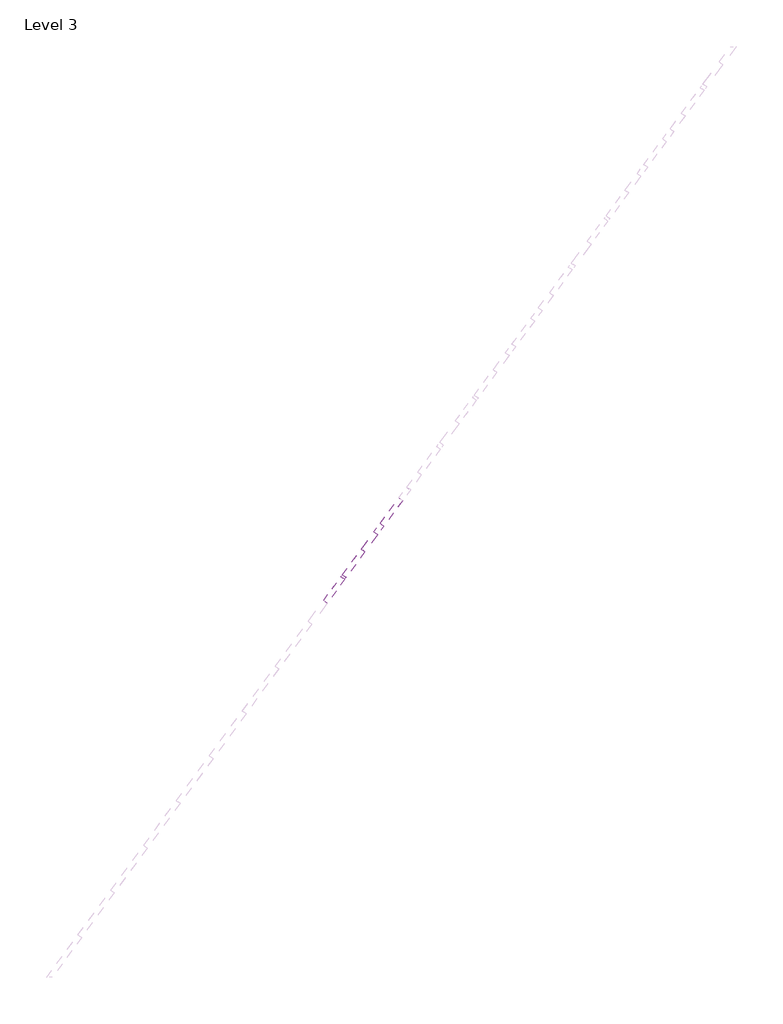
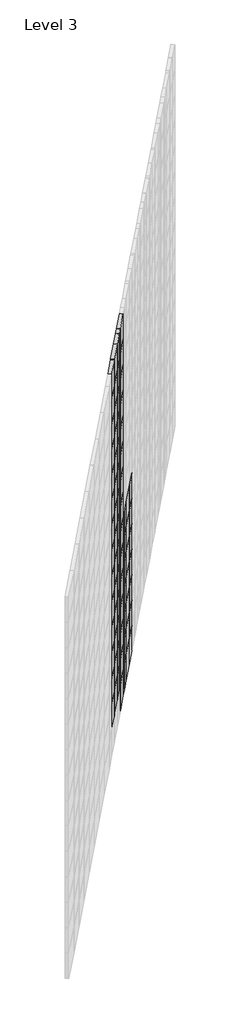
# One storey, part 4 of 9: 120 plates.
"""IFC4 building model written with IfcOpenShell, lengths in millimetres."""

import ifcopenshell
import ifcopenshell.guid

model = None  # the IFC model being written
_history = None  # IfcOwnerHistory: only IFC2X3 demands one
_inside = {}  # id of a spatial element -> (the spatial element, [elements in it])
_under = {}  # id of a project, library or spatial element -> (it, [spatial elements below it])
_declared = {}  # id of a project -> (the project, [libraries it declares])
_typed = {}  # id of a type object -> (the type object, [elements of that type])
_made_of = {}  # id of a material, layer set ... -> (it, [elements and type objects made of it])


def new_model(schema):
    """Start an empty IFC model of exactly this schema.

    Asked for "IFC4X3", IfcOpenShell would pick the latest addendum, in which some entities
    have other attributes; the version numbers below select the first issue.
    IFC2X3 requires an IfcOwnerHistory on every rooted entity: one is made here for all.
    """
    global model, _history
    if schema == "IFC4X3":
        model = ifcopenshell.file(schema_version=(4, 3, 0, 0))
    else:
        model = ifcopenshell.file(schema=schema)
    _inside.clear()
    _under.clear()
    _declared.clear()
    _typed.clear()
    _made_of.clear()
    _history = None
    if model.schema == "IFC2X3":
        org = make("IfcOrganization", Name="unknown")
        user = make(
            "IfcPersonAndOrganization",
            ThePerson=make("IfcPerson", FamilyName="unknown"),
            TheOrganization=org,
        )
        app = make(
            "IfcApplication",
            ApplicationDeveloper=org,
            Version="unknown",
            ApplicationFullName="unknown",
            ApplicationIdentifier="unknown",
        )
        _history = make(
            "IfcOwnerHistory",
            OwningUser=user,
            OwningApplication=app,
            ChangeAction="ADDED",
            CreationDate=0,
        )
    return model


def make(cls, **values):
    """One entity of the class cls with the attributes given. An attribute that is None is left unset."""
    return model.create_entity(
        cls, **{name: value for name, value in values.items() if value is not None}
    )


def rooted(cls, **values):
    """An entity with a GlobalId (a new one), such as an element, a storey or a relation."""
    return make(cls, GlobalId=ifcopenshell.guid.new(), OwnerHistory=_history, **values)


def si_unit(unit_type, name, prefix=None):
    """IfcSIUnit, for example si_unit("LENGTHUNIT", "METRE", prefix="MILLI")."""
    return make("IfcSIUnit", UnitType=unit_type, Prefix=prefix, Name=name)


def assignment(units):
    """IfcUnitAssignment: the units of a project."""
    return None if units is None else make("IfcUnitAssignment", Units=units)


def point(xyz):
    """IfcCartesianPoint."""
    return None if xyz is None else make("IfcCartesianPoint", Coordinates=xyz)


def direction(xyz):
    """IfcDirection."""
    return None if xyz is None else make("IfcDirection", DirectionRatios=xyz)


def frame(location, z_axis=None, x_axis=None):
    """IfcAxis2Placement3D, a coordinate frame: its origin and axes. An axis left out is left unset."""
    return make(
        "IfcAxis2Placement3D",
        Location=point(location),
        Axis=direction(z_axis),
        RefDirection=direction(x_axis),
    )


def origin():
    """The frame at (0, 0, 0) with its axes left unset."""
    return frame((0.0, 0.0, 0.0))


def origin_with_axes():
    """The frame at (0, 0, 0) with the z axis (0, 0, 1) and the x axis (1, 0, 0) written out."""
    return frame((0.0, 0.0, 0.0), z_axis=(0.0, 0.0, 1.0), x_axis=(1.0, 0.0, 0.0))


def place(relative_to, where):
    """IfcLocalPlacement: puts the frame where relative to a parent placement (None: the world)."""
    return make(
        "IfcLocalPlacement", PlacementRelTo=relative_to, RelativePlacement=where
    )


def context(
    kind, dimensions, precision=None, world=None, true_north=None, identifier=None
):
    """IfcGeometricRepresentationContext, for example the 3D "Model" context."""
    return make(
        "IfcGeometricRepresentationContext",
        ContextIdentifier=identifier,
        ContextType=kind,
        CoordinateSpaceDimension=dimensions,
        Precision=precision,
        WorldCoordinateSystem=world,
        TrueNorth=true_north,
    )


def project(units=None, contexts=None):
    """IfcProject with its units and contexts."""
    return rooted(
        "IfcProject",
        Name="project",
        RepresentationContexts=contexts,
        UnitsInContext=assignment(units),
    )


def spatial(cls, under=None, at=None, **own):
    """A site, building, storey or space (cls), placed at a placement, below another one or the project."""
    s = rooted(cls, ObjectPlacement=at, **own)
    if under is not None:
        _under.setdefault(under.id(), (under, []))[1].append(s)
    return s


def polyline(points):
    """IfcPolyline through the points."""
    return make("IfcPolyline", Points=[point(p) for p in points])


def outline(outer, holes=None, kind="AREA"):
    """IfcArbitraryClosedProfileDef: a profile drawn as a closed curve; with holes, ...WithVoids."""
    if holes is None:
        return make("IfcArbitraryClosedProfileDef", ProfileType=kind, OuterCurve=outer)
    return make(
        "IfcArbitraryProfileDefWithVoids",
        ProfileType=kind,
        OuterCurve=outer,
        InnerCurves=holes,
    )


def extrude(swept, where, along, depth):
    """IfcExtrudedAreaSolid: the profile swept, set in the frame where, extruded along a direction by depth."""
    return make(
        "IfcExtrudedAreaSolid",
        SweptArea=swept,
        Position=where,
        ExtrudedDirection=direction(along),
        Depth=depth,
    )


def shape(context_of_items, identifier, shape_type, items):
    """IfcShapeRepresentation: the items that make up one representation, for example the "Body"."""
    return make(
        "IfcShapeRepresentation",
        ContextOfItems=context_of_items,
        RepresentationIdentifier=identifier,
        RepresentationType=shape_type,
        Items=items,
    )


def source(mapping_origin, context_of_items, identifier, shape_type, items):
    """IfcRepresentationMap: a shape defined once, which mapped items show again and again."""
    return make(
        "IfcRepresentationMap",
        MappingOrigin=mapping_origin,
        MappedRepresentation=shape(context_of_items, identifier, shape_type, items),
    )


def transform(
    local_origin,
    x_axis=None,
    y_axis=None,
    z_axis=None,
    scale=None,
    scale2=None,
    scale3=None,
    uniform=True,
):
    """IfcCartesianTransformationOperator3D, or its non-uniform kind. x_axis, y_axis, z_axis: its Axis1, 2, 3."""
    if uniform:
        return make(
            "IfcCartesianTransformationOperator3D",
            Axis1=direction(x_axis),
            Axis2=direction(y_axis),
            LocalOrigin=point(local_origin),
            Scale=scale,
            Axis3=direction(z_axis),
        )
    return make(
        "IfcCartesianTransformationOperator3DnonUniform",
        Axis1=direction(x_axis),
        Axis2=direction(y_axis),
        LocalOrigin=point(local_origin),
        Scale=scale,
        Axis3=direction(z_axis),
        Scale2=scale2,
        Scale3=scale3,
    )


def mapped(mapping_source, mapping_target):
    """IfcMappedItem: shows the shape of a source again, moved by a transform."""
    return make(
        "IfcMappedItem", MappingSource=mapping_source, MappingTarget=mapping_target
    )


def made_of(thing, what):
    """Note that an element or type object is made of a material, layer set ...; save() writes the relation."""
    if what is not None:
        _made_of.setdefault(what.id(), (what, []))[1].append(thing)
    return thing


def element(
    cls,
    number,
    at=None,
    inside=None,
    cuts=None,
    type_object=None,
    material=None,
    context=None,
    identifier="Body",
    shape_type=None,
    held_by="IfcProductDefinitionShape",
    body=None,
    shapes=None,
    **own,
):
    """One element of the class cls, such as IfcWall. Its Tag is "e" and its number.

    at: its placement. inside: the storey or other place that contains it. cuts: it is an
    opening in that element (IfcRelVoidsElement). A single representation is given by context,
    identifier, shape_type and body (its items); several are given by shapes. held_by: the class
    of the entity that holds the representations. save() writes the other relations.
    """
    e = rooted(cls, Tag="e%d" % number, ObjectPlacement=at, **own)
    if body is not None:
        shapes = [shape(context, identifier, shape_type, body)]
    if shapes is not None:
        e.Representation = make(held_by, Representations=shapes)
    if inside is not None:
        _inside.setdefault(inside.id(), (inside, []))[1].append(e)
    if cuts is not None:
        rooted(
            "IfcRelVoidsElement", RelatingBuildingElement=cuts, RelatedOpeningElement=e
        )
    if type_object is not None:
        _typed.setdefault(type_object.id(), (type_object, []))[1].append(e)
    return made_of(e, material)


def aggregate(whole, parts):
    """IfcRelAggregates: a whole, such as a stair, and the parts it consists of."""
    return rooted("IfcRelAggregates", RelatingObject=whole, RelatedObjects=parts)


def save(model, path):
    """Write the relations noted so far, then the file.

    IfcRelAggregates (storeys below a building ...), IfcRelContainedInSpatialStructure (elements
    in a storey), IfcRelDefinesByType, IfcRelAssociatesMaterial and IfcRelDeclares: one each for
    every whole, place, type object, material and project.
    """
    for whole, parts in _under.values():
        aggregate(whole, parts)
    for where, things in _inside.values():
        rooted(
            "IfcRelContainedInSpatialStructure",
            RelatedElements=things,
            RelatingStructure=where,
        )
    for kind, things in _typed.values():
        rooted("IfcRelDefinesByType", RelatedObjects=things, RelatingType=kind)
    for what, things in _made_of.values():
        rooted("IfcRelAssociatesMaterial", RelatedObjects=things, RelatingMaterial=what)
    for by, libraries in _declared.values():
        rooted("IfcRelDeclares", RelatingContext=by, RelatedDefinitions=libraries)
    model.write(path)


def system_panel_glazed_de35cd91(model_context):
    return source(origin(), model_context, "Body", "SweptSolid", [
        extrude(outline(polyline([(6.4022601, 24.5), (-6.4022601, 24.5), (-6.4022601, 49.5), (6.4022601, 49.5), (6.4022601, 24.5)])), origin_with_axes(), (0.0, 0.0, 1.0), 200.0),
    ])


def system_panel_glazed_77252c6e(model_context):
    return source(origin(), model_context, "Body", "SweptSolid", [
        extrude(outline(polyline([(27.919021, 24.5), (-27.919021, 24.5), (-27.919021, 49.5), (27.919021, 49.5), (27.919021, 24.5)])), origin_with_axes(), (0.0, 0.0, 1.0), 200.0),
    ])


def system_panel_glazed_3dd544b4(model_context):
    return source(origin(), model_context, "Body", "SweptSolid", [
        extrude(outline(polyline([(49.4357818, 24.5), (-49.4357818, 24.5), (-49.4357818, 49.5), (49.4357818, 49.5), (49.4357818, 24.5)])), origin_with_axes(), (0.0, 0.0, 1.0), 200.0),
    ])


def system_panel_glazed_de50ea70(model_context):
    return source(origin(), model_context, "Body", "SweptSolid", [
        extrude(outline(polyline([(70.9525426, 24.5), (-70.9525426, 24.5), (-70.9525426, 49.5), (70.9525426, 49.5), (70.9525426, 24.5)])), origin_with_axes(), (0.0, 0.0, 1.0), 200.0),
    ])


def system_panel_glazed_165eaad2(model_context):
    return source(origin(), model_context, "Body", "SweptSolid", [
        extrude(outline(polyline([(78.5977399, 24.5), (-78.5977399, 24.5), (-78.5977399, 49.5), (78.5977399, 49.5), (78.5977399, 24.5)])), origin_with_axes(), (0.0, 0.0, 1.0), 200.0),
    ])


def system_panel_glazed_1ea8d406(model_context):
    return source(origin(), model_context, "Body", "SweptSolid", [
        extrude(outline(polyline([(85.0, 24.5), (-85.0, 24.5), (-85.0, 49.5), (85.0, 49.5), (85.0, 24.5)])), origin_with_axes(), (0.0, 0.0, 1.0), 200.0),
    ])


def system_panel_glazed_41e93d41(model_context):
    return source(origin(), model_context, "Body", "SweptSolid", [
        extrude(outline(polyline([(57.080979, 24.5), (-57.080979, 24.5), (-57.080979, 49.5), (57.080979, 49.5), (57.080979, 24.5)])), origin_with_axes(), (0.0, 0.0, 1.0), 200.0),
    ])


def system_panel_glazed_d81ce811(model_context):
    return source(origin(), model_context, "Body", "SweptSolid", [
        extrude(outline(polyline([(35.5642182, 24.5), (-35.5642182, 24.5), (-35.5642182, 49.5), (35.5642182, 49.5), (35.5642182, 24.5)])), origin_with_axes(), (0.0, 0.0, 1.0), 200.0),
    ])


def system_panel_glazed_acae83c8(model_context):
    return source(origin(), model_context, "Body", "SweptSolid", [
        extrude(outline(polyline([(14.0474574, 24.5), (-14.0474574, 24.5), (-14.0474574, 49.5), (14.0474574, 49.5), (14.0474574, 24.5)])), origin_with_axes(), (0.0, 0.0, 1.0), 200.0),
    ])


model = new_model("IFC4")

# Units and contexts
model_context = context("Model", 3, world=origin())
ifc_project = project(units=[si_unit("LENGTHUNIT", "METRE", prefix="MILLI")], contexts=[model_context])

# Site, building, storey
site = spatial("IfcSite", under=ifc_project)
building = spatial("IfcBuilding", under=site)
storey = spatial("IfcBuildingStorey", under=building, Name="Level 3", Elevation=22950.0)

# Plates
placement = place(None, origin())
system_panel_glazed_shape = system_panel_glazed_de35cd91(model_context)
element("IfcPlate", 1, ObjectType="System Panel : Glazed", at=placement, inside=storey, context=model_context, shape_type="MappedRepresentation", body=[
    mapped(system_panel_glazed_shape, transform((-33280.7925228, 28151.8577657, 35300.0), x_axis=(0.5920548138930122, 0.8058976965757569, 0.0), y_axis=(-0.8058976965757569, 0.5920548138930122, 0.0), z_axis=(0.0, 0.0, 1.0))),
])
element("IfcPlate", 2, ObjectType="System Panel : Glazed", at=placement, inside=storey, context=model_context, shape_type="MappedRepresentation", body=[
    mapped(system_panel_glazed_shape, transform((-33280.7925228, 28151.8577657, 35500.0), x_axis=(0.5920548138930122, 0.8058976965757569, 0.0), y_axis=(-0.8058976965757569, 0.5920548138930122, 0.0), z_axis=(0.0, 0.0, 1.0))),
])
element("IfcPlate", 3, ObjectType="System Panel : Glazed", at=placement, inside=storey, context=model_context, shape_type="MappedRepresentation", body=[
    mapped(system_panel_glazed_shape, transform((-33280.7925228, 28151.8577657, 35700.0), x_axis=(0.5920548138930122, 0.8058976965757569, 0.0), y_axis=(-0.8058976965757569, 0.5920548138930122, 0.0), z_axis=(0.0, 0.0, 1.0))),
])
element("IfcPlate", 4, ObjectType="System Panel : Glazed", at=placement, inside=storey, context=model_context, shape_type="MappedRepresentation", body=[
    mapped(system_panel_glazed_shape, transform((-33280.7925228, 28151.8577657, 35900.0), x_axis=(0.5920548138930122, 0.8058976965757569, 0.0), y_axis=(-0.8058976965757569, 0.5920548138930122, 0.0), z_axis=(0.0, 0.0, 1.0))),
])
element("IfcPlate", 5, ObjectType="System Panel : Glazed", at=placement, inside=storey, context=model_context, shape_type="MappedRepresentation", body=[
    mapped(system_panel_glazed_shape, transform((-33280.7925228, 28151.8577657, 36100.0), x_axis=(0.5920548138930122, 0.8058976965757569, 0.0), y_axis=(-0.8058976965757569, 0.5920548138930122, 0.0), z_axis=(0.0, 0.0, 1.0))),
])
element("IfcPlate", 6, ObjectType="System Panel : Glazed", at=placement, inside=storey, context=model_context, shape_type="MappedRepresentation", body=[
    mapped(system_panel_glazed_shape, transform((-33280.7925228, 28151.8577657, 36300.0), x_axis=(0.5920548138930122, 0.8058976965757569, 0.0), y_axis=(-0.8058976965757569, 0.5920548138930122, 0.0), z_axis=(0.0, 0.0, 1.0))),
])
element("IfcPlate", 7, ObjectType="System Panel : Glazed", at=placement, inside=storey, context=model_context, shape_type="MappedRepresentation", body=[
    mapped(system_panel_glazed_shape, transform((-33280.7925228, 28151.8577657, 36500.0), x_axis=(0.5920548138930122, 0.8058976965757569, 0.0), y_axis=(-0.8058976965757569, 0.5920548138930122, 0.0), z_axis=(0.0, 0.0, 1.0))),
])
element("IfcPlate", 8, ObjectType="System Panel : Glazed", at=placement, inside=storey, context=model_context, shape_type="MappedRepresentation", body=[
    mapped(system_panel_glazed_shape, transform((-33280.7925228, 28151.8577657, 36700.0), x_axis=(0.5920548138930122, 0.8058976965757569, 0.0), y_axis=(-0.8058976965757569, 0.5920548138930122, 0.0), z_axis=(0.0, 0.0, 1.0))),
])
element("IfcPlate", 9, ObjectType="System Panel : Glazed", at=placement, inside=storey, context=model_context, shape_type="MappedRepresentation", body=[
    mapped(system_panel_glazed_shape, transform((-33280.7925228, 28151.8577657, 36900.0), x_axis=(0.5920548138930122, 0.8058976965757569, 0.0), y_axis=(-0.8058976965757569, 0.5920548138930122, 0.0), z_axis=(0.0, 0.0, 1.0))),
])
element("IfcPlate", 10, ObjectType="System Panel : Glazed", at=placement, inside=storey, context=model_context, shape_type="MappedRepresentation", body=[
    mapped(system_panel_glazed_shape, transform((-33280.7925228, 28151.8577657, 37100.0), x_axis=(0.5920548138930122, 0.8058976965757569, 0.0), y_axis=(-0.8058976965757569, 0.5920548138930122, 0.0), z_axis=(0.0, 0.0, 1.0))),
])
element("IfcPlate", 11, ObjectType="System Panel : Glazed", at=placement, inside=storey, context=model_context, shape_type="MappedRepresentation", body=[
    mapped(system_panel_glazed_shape, transform((-33280.7925228, 28151.8577657, 37300.0), x_axis=(0.5920548138930122, 0.8058976965757569, 0.0), y_axis=(-0.8058976965757569, 0.5920548138930122, 0.0), z_axis=(0.0, 0.0, 1.0))),
])
element("IfcPlate", 12, ObjectType="System Panel : Glazed", at=placement, inside=storey, context=model_context, shape_type="MappedRepresentation", body=[
    mapped(system_panel_glazed_shape, transform((-33280.7925228, 28151.8577657, 37500.0), x_axis=(0.5920548138930122, 0.8058976965757569, 0.0), y_axis=(-0.8058976965757569, 0.5920548138930122, 0.0), z_axis=(0.0, 0.0, 1.0))),
])
element("IfcPlate", 13, ObjectType="System Panel : Glazed", at=placement, inside=storey, context=model_context, shape_type="MappedRepresentation", body=[
    mapped(system_panel_glazed_shape, transform((-33280.7925228, 28151.8577657, 37700.0), x_axis=(0.5920548138930122, 0.8058976965757569, 0.0), y_axis=(-0.8058976965757569, 0.5920548138930122, 0.0), z_axis=(0.0, 0.0, 1.0))),
])
element("IfcPlate", 14, ObjectType="System Panel : Glazed", at=placement, inside=storey, context=model_context, shape_type="MappedRepresentation", body=[
    mapped(system_panel_glazed_shape, transform((-33280.7925228, 28151.8577657, 37900.0), x_axis=(0.5920548138930122, 0.8058976965757569, 0.0), y_axis=(-0.8058976965757569, 0.5920548138930122, 0.0), z_axis=(0.0, 0.0, 1.0))),
])
system_panel_glazed_2_shape = system_panel_glazed_77252c6e(model_context)
element("IfcPlate", 15, ObjectType="System Panel : Glazed", at=placement, inside=storey, context=model_context, shape_type="MappedRepresentation", body=[
    mapped(system_panel_glazed_2_shape, transform((-33092.2329879, 28408.5226745, 35300.0), x_axis=(0.5920548138930122, 0.8058976965757569, 0.0), y_axis=(-0.8058976965757569, 0.5920548138930122, 0.0), z_axis=(0.0, 0.0, 1.0))),
])
element("IfcPlate", 16, ObjectType="System Panel : Glazed", at=placement, inside=storey, context=model_context, shape_type="MappedRepresentation", body=[
    mapped(system_panel_glazed_2_shape, transform((-33092.2329879, 28408.5226745, 35500.0), x_axis=(0.5920548138930122, 0.8058976965757569, 0.0), y_axis=(-0.8058976965757569, 0.5920548138930122, 0.0), z_axis=(0.0, 0.0, 1.0))),
])
element("IfcPlate", 17, ObjectType="System Panel : Glazed", at=placement, inside=storey, context=model_context, shape_type="MappedRepresentation", body=[
    mapped(system_panel_glazed_2_shape, transform((-33092.2329879, 28408.5226745, 35700.0), x_axis=(0.5920548138930122, 0.8058976965757569, 0.0), y_axis=(-0.8058976965757569, 0.5920548138930122, 0.0), z_axis=(0.0, 0.0, 1.0))),
])
element("IfcPlate", 18, ObjectType="System Panel : Glazed", at=placement, inside=storey, context=model_context, shape_type="MappedRepresentation", body=[
    mapped(system_panel_glazed_2_shape, transform((-33092.2329879, 28408.5226745, 35900.0), x_axis=(0.5920548138930122, 0.8058976965757569, 0.0), y_axis=(-0.8058976965757569, 0.5920548138930122, 0.0), z_axis=(0.0, 0.0, 1.0))),
])
element("IfcPlate", 19, ObjectType="System Panel : Glazed", at=placement, inside=storey, context=model_context, shape_type="MappedRepresentation", body=[
    mapped(system_panel_glazed_2_shape, transform((-33092.2329879, 28408.5226745, 36100.0), x_axis=(0.5920548138930122, 0.8058976965757569, 0.0), y_axis=(-0.8058976965757569, 0.5920548138930122, 0.0), z_axis=(0.0, 0.0, 1.0))),
])
element("IfcPlate", 20, ObjectType="System Panel : Glazed", at=placement, inside=storey, context=model_context, shape_type="MappedRepresentation", body=[
    mapped(system_panel_glazed_2_shape, transform((-33092.2329879, 28408.5226745, 36300.0), x_axis=(0.5920548138930122, 0.8058976965757569, 0.0), y_axis=(-0.8058976965757569, 0.5920548138930122, 0.0), z_axis=(0.0, 0.0, 1.0))),
])
element("IfcPlate", 21, ObjectType="System Panel : Glazed", at=placement, inside=storey, context=model_context, shape_type="MappedRepresentation", body=[
    mapped(system_panel_glazed_2_shape, transform((-33092.2329879, 28408.5226745, 36500.0), x_axis=(0.5920548138930122, 0.8058976965757569, 0.0), y_axis=(-0.8058976965757569, 0.5920548138930122, 0.0), z_axis=(0.0, 0.0, 1.0))),
])
element("IfcPlate", 22, ObjectType="System Panel : Glazed", at=placement, inside=storey, context=model_context, shape_type="MappedRepresentation", body=[
    mapped(system_panel_glazed_2_shape, transform((-33092.2329879, 28408.5226745, 36700.0), x_axis=(0.5920548138930122, 0.8058976965757569, 0.0), y_axis=(-0.8058976965757569, 0.5920548138930122, 0.0), z_axis=(0.0, 0.0, 1.0))),
])
element("IfcPlate", 23, ObjectType="System Panel : Glazed", at=placement, inside=storey, context=model_context, shape_type="MappedRepresentation", body=[
    mapped(system_panel_glazed_2_shape, transform((-33092.2329879, 28408.5226745, 36900.0), x_axis=(0.5920548138930122, 0.8058976965757569, 0.0), y_axis=(-0.8058976965757569, 0.5920548138930122, 0.0), z_axis=(0.0, 0.0, 1.0))),
])
element("IfcPlate", 24, ObjectType="System Panel : Glazed", at=placement, inside=storey, context=model_context, shape_type="MappedRepresentation", body=[
    mapped(system_panel_glazed_2_shape, transform((-33092.2329879, 28408.5226745, 37100.0), x_axis=(0.5920548138930122, 0.8058976965757569, 0.0), y_axis=(-0.8058976965757569, 0.5920548138930122, 0.0), z_axis=(0.0, 0.0, 1.0))),
])
element("IfcPlate", 25, ObjectType="System Panel : Glazed", at=placement, inside=storey, context=model_context, shape_type="MappedRepresentation", body=[
    mapped(system_panel_glazed_2_shape, transform((-33092.2329879, 28408.5226745, 37300.0), x_axis=(0.5920548138930122, 0.8058976965757569, 0.0), y_axis=(-0.8058976965757569, 0.5920548138930122, 0.0), z_axis=(0.0, 0.0, 1.0))),
])
element("IfcPlate", 26, ObjectType="System Panel : Glazed", at=placement, inside=storey, context=model_context, shape_type="MappedRepresentation", body=[
    mapped(system_panel_glazed_2_shape, transform((-33092.2329879, 28408.5226745, 37500.0), x_axis=(0.5920548138930122, 0.8058976965757569, 0.0), y_axis=(-0.8058976965757569, 0.5920548138930122, 0.0), z_axis=(0.0, 0.0, 1.0))),
])
element("IfcPlate", 27, ObjectType="System Panel : Glazed", at=placement, inside=storey, context=model_context, shape_type="MappedRepresentation", body=[
    mapped(system_panel_glazed_2_shape, transform((-33092.2329879, 28408.5226745, 37700.0), x_axis=(0.5920548138930122, 0.8058976965757569, 0.0), y_axis=(-0.8058976965757569, 0.5920548138930122, 0.0), z_axis=(0.0, 0.0, 1.0))),
])
element("IfcPlate", 28, ObjectType="System Panel : Glazed", at=placement, inside=storey, context=model_context, shape_type="MappedRepresentation", body=[
    mapped(system_panel_glazed_2_shape, transform((-33092.2329879, 28408.5226745, 37900.0), x_axis=(0.5920548138930122, 0.8058976965757569, 0.0), y_axis=(-0.8058976965757569, 0.5920548138930122, 0.0), z_axis=(0.0, 0.0, 1.0))),
])
system_panel_glazed_3_shape = system_panel_glazed_3dd544b4(model_context)
element("IfcPlate", 29, ObjectType="System Panel : Glazed", at=placement, inside=storey, context=model_context, shape_type="MappedRepresentation", body=[
    mapped(system_panel_glazed_3_shape, transform((-32903.673453, 28665.1875834, 35100.0), x_axis=(0.5920548138930122, 0.8058976965757569, 0.0), y_axis=(-0.8058976965757569, 0.5920548138930122, 0.0), z_axis=(0.0, 0.0, 1.0))),
])
element("IfcPlate", 30, ObjectType="System Panel : Glazed", at=placement, inside=storey, context=model_context, shape_type="MappedRepresentation", body=[
    mapped(system_panel_glazed_3_shape, transform((-32903.673453, 28665.1875834, 35300.0), x_axis=(0.5920548138930122, 0.8058976965757569, 0.0), y_axis=(-0.8058976965757569, 0.5920548138930122, 0.0), z_axis=(0.0, 0.0, 1.0))),
])
element("IfcPlate", 31, ObjectType="System Panel : Glazed", at=placement, inside=storey, context=model_context, shape_type="MappedRepresentation", body=[
    mapped(system_panel_glazed_3_shape, transform((-32903.673453, 28665.1875834, 35500.0), x_axis=(0.5920548138930122, 0.8058976965757569, 0.0), y_axis=(-0.8058976965757569, 0.5920548138930122, 0.0), z_axis=(0.0, 0.0, 1.0))),
])
element("IfcPlate", 32, ObjectType="System Panel : Glazed", at=placement, inside=storey, context=model_context, shape_type="MappedRepresentation", body=[
    mapped(system_panel_glazed_3_shape, transform((-32903.673453, 28665.1875834, 35700.0), x_axis=(0.5920548138930122, 0.8058976965757569, 0.0), y_axis=(-0.8058976965757569, 0.5920548138930122, 0.0), z_axis=(0.0, 0.0, 1.0))),
])
element("IfcPlate", 33, ObjectType="System Panel : Glazed", at=placement, inside=storey, context=model_context, shape_type="MappedRepresentation", body=[
    mapped(system_panel_glazed_3_shape, transform((-32903.673453, 28665.1875834, 35900.0), x_axis=(0.5920548138930122, 0.8058976965757569, 0.0), y_axis=(-0.8058976965757569, 0.5920548138930122, 0.0), z_axis=(0.0, 0.0, 1.0))),
])
element("IfcPlate", 34, ObjectType="System Panel : Glazed", at=placement, inside=storey, context=model_context, shape_type="MappedRepresentation", body=[
    mapped(system_panel_glazed_3_shape, transform((-32903.673453, 28665.1875834, 36100.0), x_axis=(0.5920548138930122, 0.8058976965757569, 0.0), y_axis=(-0.8058976965757569, 0.5920548138930122, 0.0), z_axis=(0.0, 0.0, 1.0))),
])
element("IfcPlate", 35, ObjectType="System Panel : Glazed", at=placement, inside=storey, context=model_context, shape_type="MappedRepresentation", body=[
    mapped(system_panel_glazed_3_shape, transform((-32903.673453, 28665.1875834, 36300.0), x_axis=(0.5920548138930122, 0.8058976965757569, 0.0), y_axis=(-0.8058976965757569, 0.5920548138930122, 0.0), z_axis=(0.0, 0.0, 1.0))),
])
system_panel_glazed_4_shape = system_panel_glazed_de50ea70(model_context)
element("IfcPlate", 36, ObjectType="System Panel : Glazed", at=placement, inside=storey, context=model_context, shape_type="MappedRepresentation", body=[
    mapped(system_panel_glazed_4_shape, transform((-32715.1139181, 28921.8524922, 35100.0), x_axis=(0.5920548138930122, 0.8058976965757569, 0.0), y_axis=(-0.8058976965757569, 0.5920548138930122, 0.0), z_axis=(0.0, 0.0, 1.0))),
])
element("IfcPlate", 37, ObjectType="System Panel : Glazed", at=placement, inside=storey, context=model_context, shape_type="MappedRepresentation", body=[
    mapped(system_panel_glazed_4_shape, transform((-32715.1139181, 28921.8524922, 35300.0), x_axis=(0.5920548138930122, 0.8058976965757569, 0.0), y_axis=(-0.8058976965757569, 0.5920548138930122, 0.0), z_axis=(0.0, 0.0, 1.0))),
])
element("IfcPlate", 38, ObjectType="System Panel : Glazed", at=placement, inside=storey, context=model_context, shape_type="MappedRepresentation", body=[
    mapped(system_panel_glazed_4_shape, transform((-32715.1139181, 28921.8524922, 35500.0), x_axis=(0.5920548138930122, 0.8058976965757569, 0.0), y_axis=(-0.8058976965757569, 0.5920548138930122, 0.0), z_axis=(0.0, 0.0, 1.0))),
])
element("IfcPlate", 39, ObjectType="System Panel : Glazed", at=placement, inside=storey, context=model_context, shape_type="MappedRepresentation", body=[
    mapped(system_panel_glazed_4_shape, transform((-32715.1139181, 28921.8524922, 35700.0), x_axis=(0.5920548138930122, 0.8058976965757569, 0.0), y_axis=(-0.8058976965757569, 0.5920548138930122, 0.0), z_axis=(0.0, 0.0, 1.0))),
])
element("IfcPlate", 40, ObjectType="System Panel : Glazed", at=placement, inside=storey, context=model_context, shape_type="MappedRepresentation", body=[
    mapped(system_panel_glazed_4_shape, transform((-32715.1139181, 28921.8524922, 35900.0), x_axis=(0.5920548138930122, 0.8058976965757569, 0.0), y_axis=(-0.8058976965757569, 0.5920548138930122, 0.0), z_axis=(0.0, 0.0, 1.0))),
])
element("IfcPlate", 41, ObjectType="System Panel : Glazed", at=placement, inside=storey, context=model_context, shape_type="MappedRepresentation", body=[
    mapped(system_panel_glazed_4_shape, transform((-32715.1139181, 28921.8524922, 36100.0), x_axis=(0.5920548138930122, 0.8058976965757569, 0.0), y_axis=(-0.8058976965757569, 0.5920548138930122, 0.0), z_axis=(0.0, 0.0, 1.0))),
])
element("IfcPlate", 42, ObjectType="System Panel : Glazed", at=placement, inside=storey, context=model_context, shape_type="MappedRepresentation", body=[
    mapped(system_panel_glazed_4_shape, transform((-32715.1139181, 28921.8524922, 36300.0), x_axis=(0.5920548138930122, 0.8058976965757569, 0.0), y_axis=(-0.8058976965757569, 0.5920548138930122, 0.0), z_axis=(0.0, 0.0, 1.0))),
])
system_panel_glazed_5_shape = system_panel_glazed_165eaad2(model_context)
element("IfcPlate", 43, ObjectType="System Panel : Glazed", at=placement, inside=storey, context=model_context, shape_type="MappedRepresentation", body=[
    mapped(system_panel_glazed_5_shape, transform((-33331.1171819, 28083.3564615, 35300.0), x_axis=(0.5920548138930122, 0.8058976965757569, 0.0), y_axis=(-0.8058976965757569, 0.5920548138930122, 0.0), z_axis=(0.0, 0.0, 1.0))),
])
element("IfcPlate", 44, ObjectType="System Panel : Glazed", at=placement, inside=storey, context=model_context, shape_type="MappedRepresentation", body=[
    mapped(system_panel_glazed_5_shape, transform((-33331.1171819, 28083.3564615, 35500.0), x_axis=(0.5920548138930122, 0.8058976965757569, 0.0), y_axis=(-0.8058976965757569, 0.5920548138930122, 0.0), z_axis=(0.0, 0.0, 1.0))),
])
element("IfcPlate", 45, ObjectType="System Panel : Glazed", at=placement, inside=storey, context=model_context, shape_type="MappedRepresentation", body=[
    mapped(system_panel_glazed_5_shape, transform((-33331.1171819, 28083.3564615, 35700.0), x_axis=(0.5920548138930122, 0.8058976965757569, 0.0), y_axis=(-0.8058976965757569, 0.5920548138930122, 0.0), z_axis=(0.0, 0.0, 1.0))),
])
element("IfcPlate", 46, ObjectType="System Panel : Glazed", at=placement, inside=storey, context=model_context, shape_type="MappedRepresentation", body=[
    mapped(system_panel_glazed_5_shape, transform((-33331.1171819, 28083.3564615, 35900.0), x_axis=(0.5920548138930122, 0.8058976965757569, 0.0), y_axis=(-0.8058976965757569, 0.5920548138930122, 0.0), z_axis=(0.0, 0.0, 1.0))),
])
element("IfcPlate", 47, ObjectType="System Panel : Glazed", at=placement, inside=storey, context=model_context, shape_type="MappedRepresentation", body=[
    mapped(system_panel_glazed_5_shape, transform((-33331.1171819, 28083.3564615, 36100.0), x_axis=(0.5920548138930122, 0.8058976965757569, 0.0), y_axis=(-0.8058976965757569, 0.5920548138930122, 0.0), z_axis=(0.0, 0.0, 1.0))),
])
element("IfcPlate", 48, ObjectType="System Panel : Glazed", at=placement, inside=storey, context=model_context, shape_type="MappedRepresentation", body=[
    mapped(system_panel_glazed_5_shape, transform((-33331.1171819, 28083.3564615, 36300.0), x_axis=(0.5920548138930122, 0.8058976965757569, 0.0), y_axis=(-0.8058976965757569, 0.5920548138930122, 0.0), z_axis=(0.0, 0.0, 1.0))),
])
element("IfcPlate", 49, ObjectType="System Panel : Glazed", at=placement, inside=storey, context=model_context, shape_type="MappedRepresentation", body=[
    mapped(system_panel_glazed_5_shape, transform((-33331.1171819, 28083.3564615, 36500.0), x_axis=(0.5920548138930122, 0.8058976965757569, 0.0), y_axis=(-0.8058976965757569, 0.5920548138930122, 0.0), z_axis=(0.0, 0.0, 1.0))),
])
element("IfcPlate", 50, ObjectType="System Panel : Glazed", at=placement, inside=storey, context=model_context, shape_type="MappedRepresentation", body=[
    mapped(system_panel_glazed_5_shape, transform((-33331.1171819, 28083.3564615, 36700.0), x_axis=(0.5920548138930122, 0.8058976965757569, 0.0), y_axis=(-0.8058976965757569, 0.5920548138930122, 0.0), z_axis=(0.0, 0.0, 1.0))),
])
element("IfcPlate", 51, ObjectType="System Panel : Glazed", at=placement, inside=storey, context=model_context, shape_type="MappedRepresentation", body=[
    mapped(system_panel_glazed_5_shape, transform((-33331.1171819, 28083.3564615, 36900.0), x_axis=(0.5920548138930122, 0.8058976965757569, 0.0), y_axis=(-0.8058976965757569, 0.5920548138930122, 0.0), z_axis=(0.0, 0.0, 1.0))),
])
element("IfcPlate", 52, ObjectType="System Panel : Glazed", at=placement, inside=storey, context=model_context, shape_type="MappedRepresentation", body=[
    mapped(system_panel_glazed_5_shape, transform((-33331.1171819, 28083.3564615, 37100.0), x_axis=(0.5920548138930122, 0.8058976965757569, 0.0), y_axis=(-0.8058976965757569, 0.5920548138930122, 0.0), z_axis=(0.0, 0.0, 1.0))),
])
element("IfcPlate", 53, ObjectType="System Panel : Glazed", at=placement, inside=storey, context=model_context, shape_type="MappedRepresentation", body=[
    mapped(system_panel_glazed_5_shape, transform((-33331.1171819, 28083.3564615, 37300.0), x_axis=(0.5920548138930122, 0.8058976965757569, 0.0), y_axis=(-0.8058976965757569, 0.5920548138930122, 0.0), z_axis=(0.0, 0.0, 1.0))),
])
element("IfcPlate", 54, ObjectType="System Panel : Glazed", at=placement, inside=storey, context=model_context, shape_type="MappedRepresentation", body=[
    mapped(system_panel_glazed_5_shape, transform((-33331.1171819, 28083.3564615, 37500.0), x_axis=(0.5920548138930122, 0.8058976965757569, 0.0), y_axis=(-0.8058976965757569, 0.5920548138930122, 0.0), z_axis=(0.0, 0.0, 1.0))),
])
element("IfcPlate", 55, ObjectType="System Panel : Glazed", at=placement, inside=storey, context=model_context, shape_type="MappedRepresentation", body=[
    mapped(system_panel_glazed_5_shape, transform((-33331.1171819, 28083.3564615, 37700.0), x_axis=(0.5920548138930122, 0.8058976965757569, 0.0), y_axis=(-0.8058976965757569, 0.5920548138930122, 0.0), z_axis=(0.0, 0.0, 1.0))),
])
element("IfcPlate", 56, ObjectType="System Panel : Glazed", at=placement, inside=storey, context=model_context, shape_type="MappedRepresentation", body=[
    mapped(system_panel_glazed_5_shape, transform((-33331.1171819, 28083.3564615, 37900.0), x_axis=(0.5920548138930122, 0.8058976965757569, 0.0), y_axis=(-0.8058976965757569, 0.5920548138930122, 0.0), z_axis=(0.0, 0.0, 1.0))),
])
system_panel_glazed_6_shape = system_panel_glazed_1ea8d406(model_context)
element("IfcPlate", 57, ObjectType="System Panel : Glazed", at=placement, inside=storey, context=model_context, shape_type="MappedRepresentation", body=[
    mapped(system_panel_glazed_6_shape, transform((-33025.3787379, 28499.5238534, 35100.0), x_axis=(0.5920548138930122, 0.8058976965757569, 0.0), y_axis=(-0.8058976965757569, 0.5920548138930122, 0.0), z_axis=(0.0, 0.0, 1.0))),
])
element("IfcPlate", 58, ObjectType="System Panel : Glazed", at=placement, inside=storey, context=model_context, shape_type="MappedRepresentation", body=[
    mapped(system_panel_glazed_6_shape, transform((-32824.0801012, 28773.5290702, 35100.0), x_axis=(0.5920548138930122, 0.8058976965757569, 0.0), y_axis=(-0.8058976965757569, 0.5920548138930122, 0.0), z_axis=(0.0, 0.0, 1.0))),
])
element("IfcPlate", 59, ObjectType="System Panel : Glazed", at=placement, inside=storey, context=model_context, shape_type="MappedRepresentation", body=[
    mapped(system_panel_glazed_6_shape, transform((-33226.6773747, 28225.5186366, 35300.0), x_axis=(0.5920548138930122, 0.8058976965757569, 0.0), y_axis=(-0.8058976965757569, 0.5920548138930122, 0.0), z_axis=(0.0, 0.0, 1.0))),
])
element("IfcPlate", 60, ObjectType="System Panel : Glazed", at=placement, inside=storey, context=model_context, shape_type="MappedRepresentation", body=[
    mapped(system_panel_glazed_6_shape, transform((-33025.3787379, 28499.5238534, 35300.0), x_axis=(0.5920548138930122, 0.8058976965757569, 0.0), y_axis=(-0.8058976965757569, 0.5920548138930122, 0.0), z_axis=(0.0, 0.0, 1.0))),
])
element("IfcPlate", 61, ObjectType="System Panel : Glazed", at=placement, inside=storey, context=model_context, shape_type="MappedRepresentation", body=[
    mapped(system_panel_glazed_6_shape, transform((-32824.0801012, 28773.5290702, 35300.0), x_axis=(0.5920548138930122, 0.8058976965757569, 0.0), y_axis=(-0.8058976965757569, 0.5920548138930122, 0.0), z_axis=(0.0, 0.0, 1.0))),
])
element("IfcPlate", 62, ObjectType="System Panel : Glazed", at=placement, inside=storey, context=model_context, shape_type="MappedRepresentation", body=[
    mapped(system_panel_glazed_6_shape, transform((-33226.6773747, 28225.5186366, 35500.0), x_axis=(0.5920548138930122, 0.8058976965757569, 0.0), y_axis=(-0.8058976965757569, 0.5920548138930122, 0.0), z_axis=(0.0, 0.0, 1.0))),
])
element("IfcPlate", 63, ObjectType="System Panel : Glazed", at=placement, inside=storey, context=model_context, shape_type="MappedRepresentation", body=[
    mapped(system_panel_glazed_6_shape, transform((-33025.3787379, 28499.5238534, 35500.0), x_axis=(0.5920548138930122, 0.8058976965757569, 0.0), y_axis=(-0.8058976965757569, 0.5920548138930122, 0.0), z_axis=(0.0, 0.0, 1.0))),
])
element("IfcPlate", 64, ObjectType="System Panel : Glazed", at=placement, inside=storey, context=model_context, shape_type="MappedRepresentation", body=[
    mapped(system_panel_glazed_6_shape, transform((-32824.0801012, 28773.5290702, 35500.0), x_axis=(0.5920548138930122, 0.8058976965757569, 0.0), y_axis=(-0.8058976965757569, 0.5920548138930122, 0.0), z_axis=(0.0, 0.0, 1.0))),
])
element("IfcPlate", 65, ObjectType="System Panel : Glazed", at=placement, inside=storey, context=model_context, shape_type="MappedRepresentation", body=[
    mapped(system_panel_glazed_6_shape, transform((-33226.6773747, 28225.5186366, 35700.0), x_axis=(0.5920548138930122, 0.8058976965757569, 0.0), y_axis=(-0.8058976965757569, 0.5920548138930122, 0.0), z_axis=(0.0, 0.0, 1.0))),
])
element("IfcPlate", 66, ObjectType="System Panel : Glazed", at=placement, inside=storey, context=model_context, shape_type="MappedRepresentation", body=[
    mapped(system_panel_glazed_6_shape, transform((-33025.3787379, 28499.5238534, 35700.0), x_axis=(0.5920548138930122, 0.8058976965757569, 0.0), y_axis=(-0.8058976965757569, 0.5920548138930122, 0.0), z_axis=(0.0, 0.0, 1.0))),
])
element("IfcPlate", 67, ObjectType="System Panel : Glazed", at=placement, inside=storey, context=model_context, shape_type="MappedRepresentation", body=[
    mapped(system_panel_glazed_6_shape, transform((-32824.0801012, 28773.5290702, 35700.0), x_axis=(0.5920548138930122, 0.8058976965757569, 0.0), y_axis=(-0.8058976965757569, 0.5920548138930122, 0.0), z_axis=(0.0, 0.0, 1.0))),
])
element("IfcPlate", 68, ObjectType="System Panel : Glazed", at=placement, inside=storey, context=model_context, shape_type="MappedRepresentation", body=[
    mapped(system_panel_glazed_6_shape, transform((-33226.6773747, 28225.5186366, 35900.0), x_axis=(0.5920548138930122, 0.8058976965757569, 0.0), y_axis=(-0.8058976965757569, 0.5920548138930122, 0.0), z_axis=(0.0, 0.0, 1.0))),
])
element("IfcPlate", 69, ObjectType="System Panel : Glazed", at=placement, inside=storey, context=model_context, shape_type="MappedRepresentation", body=[
    mapped(system_panel_glazed_6_shape, transform((-33025.3787379, 28499.5238534, 35900.0), x_axis=(0.5920548138930122, 0.8058976965757569, 0.0), y_axis=(-0.8058976965757569, 0.5920548138930122, 0.0), z_axis=(0.0, 0.0, 1.0))),
])
element("IfcPlate", 70, ObjectType="System Panel : Glazed", at=placement, inside=storey, context=model_context, shape_type="MappedRepresentation", body=[
    mapped(system_panel_glazed_6_shape, transform((-32824.0801012, 28773.5290702, 35900.0), x_axis=(0.5920548138930122, 0.8058976965757569, 0.0), y_axis=(-0.8058976965757569, 0.5920548138930122, 0.0), z_axis=(0.0, 0.0, 1.0))),
])
element("IfcPlate", 71, ObjectType="System Panel : Glazed", at=placement, inside=storey, context=model_context, shape_type="MappedRepresentation", body=[
    mapped(system_panel_glazed_6_shape, transform((-33226.6773747, 28225.5186366, 36100.0), x_axis=(0.5920548138930122, 0.8058976965757569, 0.0), y_axis=(-0.8058976965757569, 0.5920548138930122, 0.0), z_axis=(0.0, 0.0, 1.0))),
])
element("IfcPlate", 72, ObjectType="System Panel : Glazed", at=placement, inside=storey, context=model_context, shape_type="MappedRepresentation", body=[
    mapped(system_panel_glazed_6_shape, transform((-33025.3787379, 28499.5238534, 36100.0), x_axis=(0.5920548138930122, 0.8058976965757569, 0.0), y_axis=(-0.8058976965757569, 0.5920548138930122, 0.0), z_axis=(0.0, 0.0, 1.0))),
])
element("IfcPlate", 73, ObjectType="System Panel : Glazed", at=placement, inside=storey, context=model_context, shape_type="MappedRepresentation", body=[
    mapped(system_panel_glazed_6_shape, transform((-32824.0801012, 28773.5290702, 36100.0), x_axis=(0.5920548138930122, 0.8058976965757569, 0.0), y_axis=(-0.8058976965757569, 0.5920548138930122, 0.0), z_axis=(0.0, 0.0, 1.0))),
])
element("IfcPlate", 74, ObjectType="System Panel : Glazed", at=placement, inside=storey, context=model_context, shape_type="MappedRepresentation", body=[
    mapped(system_panel_glazed_6_shape, transform((-33226.6773747, 28225.5186366, 36300.0), x_axis=(0.5920548138930122, 0.8058976965757569, 0.0), y_axis=(-0.8058976965757569, 0.5920548138930122, 0.0), z_axis=(0.0, 0.0, 1.0))),
])
element("IfcPlate", 75, ObjectType="System Panel : Glazed", at=placement, inside=storey, context=model_context, shape_type="MappedRepresentation", body=[
    mapped(system_panel_glazed_6_shape, transform((-33025.3787379, 28499.5238534, 36300.0), x_axis=(0.5920548138930122, 0.8058976965757569, 0.0), y_axis=(-0.8058976965757569, 0.5920548138930122, 0.0), z_axis=(0.0, 0.0, 1.0))),
])
element("IfcPlate", 76, ObjectType="System Panel : Glazed", at=placement, inside=storey, context=model_context, shape_type="MappedRepresentation", body=[
    mapped(system_panel_glazed_6_shape, transform((-32824.0801012, 28773.5290702, 36300.0), x_axis=(0.5920548138930122, 0.8058976965757569, 0.0), y_axis=(-0.8058976965757569, 0.5920548138930122, 0.0), z_axis=(0.0, 0.0, 1.0))),
])
element("IfcPlate", 77, ObjectType="System Panel : Glazed", at=placement, inside=storey, context=model_context, shape_type="MappedRepresentation", body=[
    mapped(system_panel_glazed_6_shape, transform((-33226.6773747, 28225.5186366, 36500.0), x_axis=(0.5920548138930122, 0.8058976965757569, 0.0), y_axis=(-0.8058976965757569, 0.5920548138930122, 0.0), z_axis=(0.0, 0.0, 1.0))),
])
element("IfcPlate", 78, ObjectType="System Panel : Glazed", at=placement, inside=storey, context=model_context, shape_type="MappedRepresentation", body=[
    mapped(system_panel_glazed_6_shape, transform((-33025.3787379, 28499.5238534, 36500.0), x_axis=(0.5920548138930122, 0.8058976965757569, 0.0), y_axis=(-0.8058976965757569, 0.5920548138930122, 0.0), z_axis=(0.0, 0.0, 1.0))),
])
element("IfcPlate", 79, ObjectType="System Panel : Glazed", at=placement, inside=storey, context=model_context, shape_type="MappedRepresentation", body=[
    mapped(system_panel_glazed_6_shape, transform((-33226.6773747, 28225.5186366, 36700.0), x_axis=(0.5920548138930122, 0.8058976965757569, 0.0), y_axis=(-0.8058976965757569, 0.5920548138930122, 0.0), z_axis=(0.0, 0.0, 1.0))),
])
element("IfcPlate", 80, ObjectType="System Panel : Glazed", at=placement, inside=storey, context=model_context, shape_type="MappedRepresentation", body=[
    mapped(system_panel_glazed_6_shape, transform((-33025.3787379, 28499.5238534, 36700.0), x_axis=(0.5920548138930122, 0.8058976965757569, 0.0), y_axis=(-0.8058976965757569, 0.5920548138930122, 0.0), z_axis=(0.0, 0.0, 1.0))),
])
element("IfcPlate", 81, ObjectType="System Panel : Glazed", at=placement, inside=storey, context=model_context, shape_type="MappedRepresentation", body=[
    mapped(system_panel_glazed_6_shape, transform((-33226.6773747, 28225.5186366, 36900.0), x_axis=(0.5920548138930122, 0.8058976965757569, 0.0), y_axis=(-0.8058976965757569, 0.5920548138930122, 0.0), z_axis=(0.0, 0.0, 1.0))),
])
element("IfcPlate", 82, ObjectType="System Panel : Glazed", at=placement, inside=storey, context=model_context, shape_type="MappedRepresentation", body=[
    mapped(system_panel_glazed_6_shape, transform((-33025.3787379, 28499.5238534, 36900.0), x_axis=(0.5920548138930122, 0.8058976965757569, 0.0), y_axis=(-0.8058976965757569, 0.5920548138930122, 0.0), z_axis=(0.0, 0.0, 1.0))),
])
element("IfcPlate", 83, ObjectType="System Panel : Glazed", at=placement, inside=storey, context=model_context, shape_type="MappedRepresentation", body=[
    mapped(system_panel_glazed_6_shape, transform((-33226.6773747, 28225.5186366, 37100.0), x_axis=(0.5920548138930122, 0.8058976965757569, 0.0), y_axis=(-0.8058976965757569, 0.5920548138930122, 0.0), z_axis=(0.0, 0.0, 1.0))),
])
element("IfcPlate", 84, ObjectType="System Panel : Glazed", at=placement, inside=storey, context=model_context, shape_type="MappedRepresentation", body=[
    mapped(system_panel_glazed_6_shape, transform((-33025.3787379, 28499.5238534, 37100.0), x_axis=(0.5920548138930122, 0.8058976965757569, 0.0), y_axis=(-0.8058976965757569, 0.5920548138930122, 0.0), z_axis=(0.0, 0.0, 1.0))),
])
element("IfcPlate", 85, ObjectType="System Panel : Glazed", at=placement, inside=storey, context=model_context, shape_type="MappedRepresentation", body=[
    mapped(system_panel_glazed_6_shape, transform((-33226.6773747, 28225.5186366, 37300.0), x_axis=(0.5920548138930122, 0.8058976965757569, 0.0), y_axis=(-0.8058976965757569, 0.5920548138930122, 0.0), z_axis=(0.0, 0.0, 1.0))),
])
element("IfcPlate", 86, ObjectType="System Panel : Glazed", at=placement, inside=storey, context=model_context, shape_type="MappedRepresentation", body=[
    mapped(system_panel_glazed_6_shape, transform((-33025.3787379, 28499.5238534, 37300.0), x_axis=(0.5920548138930122, 0.8058976965757569, 0.0), y_axis=(-0.8058976965757569, 0.5920548138930122, 0.0), z_axis=(0.0, 0.0, 1.0))),
])
element("IfcPlate", 87, ObjectType="System Panel : Glazed", at=placement, inside=storey, context=model_context, shape_type="MappedRepresentation", body=[
    mapped(system_panel_glazed_6_shape, transform((-33226.6773747, 28225.5186366, 37500.0), x_axis=(0.5920548138930122, 0.8058976965757569, 0.0), y_axis=(-0.8058976965757569, 0.5920548138930122, 0.0), z_axis=(0.0, 0.0, 1.0))),
])
element("IfcPlate", 88, ObjectType="System Panel : Glazed", at=placement, inside=storey, context=model_context, shape_type="MappedRepresentation", body=[
    mapped(system_panel_glazed_6_shape, transform((-33025.3787379, 28499.5238534, 37500.0), x_axis=(0.5920548138930122, 0.8058976965757569, 0.0), y_axis=(-0.8058976965757569, 0.5920548138930122, 0.0), z_axis=(0.0, 0.0, 1.0))),
])
element("IfcPlate", 89, ObjectType="System Panel : Glazed", at=placement, inside=storey, context=model_context, shape_type="MappedRepresentation", body=[
    mapped(system_panel_glazed_6_shape, transform((-33226.6773747, 28225.5186366, 37700.0), x_axis=(0.5920548138930122, 0.8058976965757569, 0.0), y_axis=(-0.8058976965757569, 0.5920548138930122, 0.0), z_axis=(0.0, 0.0, 1.0))),
])
element("IfcPlate", 90, ObjectType="System Panel : Glazed", at=placement, inside=storey, context=model_context, shape_type="MappedRepresentation", body=[
    mapped(system_panel_glazed_6_shape, transform((-33025.3787379, 28499.5238534, 37700.0), x_axis=(0.5920548138930122, 0.8058976965757569, 0.0), y_axis=(-0.8058976965757569, 0.5920548138930122, 0.0), z_axis=(0.0, 0.0, 1.0))),
])
element("IfcPlate", 91, ObjectType="System Panel : Glazed", at=placement, inside=storey, context=model_context, shape_type="MappedRepresentation", body=[
    mapped(system_panel_glazed_6_shape, transform((-33226.6773747, 28225.5186366, 37900.0), x_axis=(0.5920548138930122, 0.8058976965757569, 0.0), y_axis=(-0.8058976965757569, 0.5920548138930122, 0.0), z_axis=(0.0, 0.0, 1.0))),
])
element("IfcPlate", 92, ObjectType="System Panel : Glazed", at=placement, inside=storey, context=model_context, shape_type="MappedRepresentation", body=[
    mapped(system_panel_glazed_6_shape, transform((-33025.3787379, 28499.5238534, 37900.0), x_axis=(0.5920548138930122, 0.8058976965757569, 0.0), y_axis=(-0.8058976965757569, 0.5920548138930122, 0.0), z_axis=(0.0, 0.0, 1.0))),
])
system_panel_glazed_7_shape = system_panel_glazed_41e93d41(model_context)
element("IfcPlate", 93, ObjectType="System Panel : Glazed", at=placement, inside=storey, context=model_context, shape_type="MappedRepresentation", body=[
    mapped(system_panel_glazed_7_shape, transform((-33142.5576471, 28340.0213703, 35300.0), x_axis=(0.5920548138930122, 0.8058976965757569, 0.0), y_axis=(-0.8058976965757569, 0.5920548138930122, 0.0), z_axis=(0.0, 0.0, 1.0))),
])
element("IfcPlate", 94, ObjectType="System Panel : Glazed", at=placement, inside=storey, context=model_context, shape_type="MappedRepresentation", body=[
    mapped(system_panel_glazed_7_shape, transform((-33142.5576471, 28340.0213703, 35500.0), x_axis=(0.5920548138930122, 0.8058976965757569, 0.0), y_axis=(-0.8058976965757569, 0.5920548138930122, 0.0), z_axis=(0.0, 0.0, 1.0))),
])
element("IfcPlate", 95, ObjectType="System Panel : Glazed", at=placement, inside=storey, context=model_context, shape_type="MappedRepresentation", body=[
    mapped(system_panel_glazed_7_shape, transform((-33142.5576471, 28340.0213703, 35700.0), x_axis=(0.5920548138930122, 0.8058976965757569, 0.0), y_axis=(-0.8058976965757569, 0.5920548138930122, 0.0), z_axis=(0.0, 0.0, 1.0))),
])
element("IfcPlate", 96, ObjectType="System Panel : Glazed", at=placement, inside=storey, context=model_context, shape_type="MappedRepresentation", body=[
    mapped(system_panel_glazed_7_shape, transform((-33142.5576471, 28340.0213703, 35900.0), x_axis=(0.5920548138930122, 0.8058976965757569, 0.0), y_axis=(-0.8058976965757569, 0.5920548138930122, 0.0), z_axis=(0.0, 0.0, 1.0))),
])
element("IfcPlate", 97, ObjectType="System Panel : Glazed", at=placement, inside=storey, context=model_context, shape_type="MappedRepresentation", body=[
    mapped(system_panel_glazed_7_shape, transform((-33142.5576471, 28340.0213703, 36100.0), x_axis=(0.5920548138930122, 0.8058976965757569, 0.0), y_axis=(-0.8058976965757569, 0.5920548138930122, 0.0), z_axis=(0.0, 0.0, 1.0))),
])
element("IfcPlate", 98, ObjectType="System Panel : Glazed", at=placement, inside=storey, context=model_context, shape_type="MappedRepresentation", body=[
    mapped(system_panel_glazed_7_shape, transform((-33142.5576471, 28340.0213703, 36300.0), x_axis=(0.5920548138930122, 0.8058976965757569, 0.0), y_axis=(-0.8058976965757569, 0.5920548138930122, 0.0), z_axis=(0.0, 0.0, 1.0))),
])
element("IfcPlate", 99, ObjectType="System Panel : Glazed", at=placement, inside=storey, context=model_context, shape_type="MappedRepresentation", body=[
    mapped(system_panel_glazed_7_shape, transform((-33142.5576471, 28340.0213703, 36500.0), x_axis=(0.5920548138930122, 0.8058976965757569, 0.0), y_axis=(-0.8058976965757569, 0.5920548138930122, 0.0), z_axis=(0.0, 0.0, 1.0))),
])
element("IfcPlate", 100, ObjectType="System Panel : Glazed", at=placement, inside=storey, context=model_context, shape_type="MappedRepresentation", body=[
    mapped(system_panel_glazed_7_shape, transform((-33142.5576471, 28340.0213703, 36700.0), x_axis=(0.5920548138930122, 0.8058976965757569, 0.0), y_axis=(-0.8058976965757569, 0.5920548138930122, 0.0), z_axis=(0.0, 0.0, 1.0))),
])
element("IfcPlate", 101, ObjectType="System Panel : Glazed", at=placement, inside=storey, context=model_context, shape_type="MappedRepresentation", body=[
    mapped(system_panel_glazed_7_shape, transform((-33142.5576471, 28340.0213703, 36900.0), x_axis=(0.5920548138930122, 0.8058976965757569, 0.0), y_axis=(-0.8058976965757569, 0.5920548138930122, 0.0), z_axis=(0.0, 0.0, 1.0))),
])
element("IfcPlate", 102, ObjectType="System Panel : Glazed", at=placement, inside=storey, context=model_context, shape_type="MappedRepresentation", body=[
    mapped(system_panel_glazed_7_shape, transform((-33142.5576471, 28340.0213703, 37100.0), x_axis=(0.5920548138930122, 0.8058976965757569, 0.0), y_axis=(-0.8058976965757569, 0.5920548138930122, 0.0), z_axis=(0.0, 0.0, 1.0))),
])
element("IfcPlate", 103, ObjectType="System Panel : Glazed", at=placement, inside=storey, context=model_context, shape_type="MappedRepresentation", body=[
    mapped(system_panel_glazed_7_shape, transform((-33142.5576471, 28340.0213703, 37300.0), x_axis=(0.5920548138930122, 0.8058976965757569, 0.0), y_axis=(-0.8058976965757569, 0.5920548138930122, 0.0), z_axis=(0.0, 0.0, 1.0))),
])
element("IfcPlate", 104, ObjectType="System Panel : Glazed", at=placement, inside=storey, context=model_context, shape_type="MappedRepresentation", body=[
    mapped(system_panel_glazed_7_shape, transform((-33142.5576471, 28340.0213703, 37500.0), x_axis=(0.5920548138930122, 0.8058976965757569, 0.0), y_axis=(-0.8058976965757569, 0.5920548138930122, 0.0), z_axis=(0.0, 0.0, 1.0))),
])
element("IfcPlate", 105, ObjectType="System Panel : Glazed", at=placement, inside=storey, context=model_context, shape_type="MappedRepresentation", body=[
    mapped(system_panel_glazed_7_shape, transform((-33142.5576471, 28340.0213703, 37700.0), x_axis=(0.5920548138930122, 0.8058976965757569, 0.0), y_axis=(-0.8058976965757569, 0.5920548138930122, 0.0), z_axis=(0.0, 0.0, 1.0))),
])
element("IfcPlate", 106, ObjectType="System Panel : Glazed", at=placement, inside=storey, context=model_context, shape_type="MappedRepresentation", body=[
    mapped(system_panel_glazed_7_shape, transform((-33142.5576471, 28340.0213703, 37900.0), x_axis=(0.5920548138930122, 0.8058976965757569, 0.0), y_axis=(-0.8058976965757569, 0.5920548138930122, 0.0), z_axis=(0.0, 0.0, 1.0))),
])
system_panel_glazed_8_shape = system_panel_glazed_d81ce811(model_context)
element("IfcPlate", 107, ObjectType="System Panel : Glazed", at=placement, inside=storey, context=model_context, shape_type="MappedRepresentation", body=[
    mapped(system_panel_glazed_8_shape, transform((-32953.9981122, 28596.6862791, 35100.0), x_axis=(0.5920548138930122, 0.8058976965757569, 0.0), y_axis=(-0.8058976965757569, 0.5920548138930122, 0.0), z_axis=(0.0, 0.0, 1.0))),
])
element("IfcPlate", 108, ObjectType="System Panel : Glazed", at=placement, inside=storey, context=model_context, shape_type="MappedRepresentation", body=[
    mapped(system_panel_glazed_8_shape, transform((-32953.9981122, 28596.6862791, 35300.0), x_axis=(0.5920548138930122, 0.8058976965757569, 0.0), y_axis=(-0.8058976965757569, 0.5920548138930122, 0.0), z_axis=(0.0, 0.0, 1.0))),
])
element("IfcPlate", 109, ObjectType="System Panel : Glazed", at=placement, inside=storey, context=model_context, shape_type="MappedRepresentation", body=[
    mapped(system_panel_glazed_8_shape, transform((-32953.9981122, 28596.6862791, 35500.0), x_axis=(0.5920548138930122, 0.8058976965757569, 0.0), y_axis=(-0.8058976965757569, 0.5920548138930122, 0.0), z_axis=(0.0, 0.0, 1.0))),
])
element("IfcPlate", 110, ObjectType="System Panel : Glazed", at=placement, inside=storey, context=model_context, shape_type="MappedRepresentation", body=[
    mapped(system_panel_glazed_8_shape, transform((-32953.9981122, 28596.6862791, 35700.0), x_axis=(0.5920548138930122, 0.8058976965757569, 0.0), y_axis=(-0.8058976965757569, 0.5920548138930122, 0.0), z_axis=(0.0, 0.0, 1.0))),
])
element("IfcPlate", 111, ObjectType="System Panel : Glazed", at=placement, inside=storey, context=model_context, shape_type="MappedRepresentation", body=[
    mapped(system_panel_glazed_8_shape, transform((-32953.9981122, 28596.6862791, 35900.0), x_axis=(0.5920548138930122, 0.8058976965757569, 0.0), y_axis=(-0.8058976965757569, 0.5920548138930122, 0.0), z_axis=(0.0, 0.0, 1.0))),
])
element("IfcPlate", 112, ObjectType="System Panel : Glazed", at=placement, inside=storey, context=model_context, shape_type="MappedRepresentation", body=[
    mapped(system_panel_glazed_8_shape, transform((-32953.9981122, 28596.6862791, 36100.0), x_axis=(0.5920548138930122, 0.8058976965757569, 0.0), y_axis=(-0.8058976965757569, 0.5920548138930122, 0.0), z_axis=(0.0, 0.0, 1.0))),
])
element("IfcPlate", 113, ObjectType="System Panel : Glazed", at=placement, inside=storey, context=model_context, shape_type="MappedRepresentation", body=[
    mapped(system_panel_glazed_8_shape, transform((-32953.9981122, 28596.6862791, 36300.0), x_axis=(0.5920548138930122, 0.8058976965757569, 0.0), y_axis=(-0.8058976965757569, 0.5920548138930122, 0.0), z_axis=(0.0, 0.0, 1.0))),
])
system_panel_glazed_9_shape = system_panel_glazed_acae83c8(model_context)
element("IfcPlate", 114, ObjectType="System Panel : Glazed", at=placement, inside=storey, context=model_context, shape_type="MappedRepresentation", body=[
    mapped(system_panel_glazed_9_shape, transform((-32765.4385773, 28853.351188, 35100.0), x_axis=(0.5920548138930122, 0.8058976965757569, 0.0), y_axis=(-0.8058976965757569, 0.5920548138930122, 0.0), z_axis=(0.0, 0.0, 1.0))),
])
element("IfcPlate", 115, ObjectType="System Panel : Glazed", at=placement, inside=storey, context=model_context, shape_type="MappedRepresentation", body=[
    mapped(system_panel_glazed_9_shape, transform((-32765.4385773, 28853.351188, 35300.0), x_axis=(0.5920548138930122, 0.8058976965757569, 0.0), y_axis=(-0.8058976965757569, 0.5920548138930122, 0.0), z_axis=(0.0, 0.0, 1.0))),
])
element("IfcPlate", 116, ObjectType="System Panel : Glazed", at=placement, inside=storey, context=model_context, shape_type="MappedRepresentation", body=[
    mapped(system_panel_glazed_9_shape, transform((-32765.4385773, 28853.351188, 35500.0), x_axis=(0.5920548138930122, 0.8058976965757569, 0.0), y_axis=(-0.8058976965757569, 0.5920548138930122, 0.0), z_axis=(0.0, 0.0, 1.0))),
])
element("IfcPlate", 117, ObjectType="System Panel : Glazed", at=placement, inside=storey, context=model_context, shape_type="MappedRepresentation", body=[
    mapped(system_panel_glazed_9_shape, transform((-32765.4385773, 28853.351188, 35700.0), x_axis=(0.5920548138930122, 0.8058976965757569, 0.0), y_axis=(-0.8058976965757569, 0.5920548138930122, 0.0), z_axis=(0.0, 0.0, 1.0))),
])
element("IfcPlate", 118, ObjectType="System Panel : Glazed", at=placement, inside=storey, context=model_context, shape_type="MappedRepresentation", body=[
    mapped(system_panel_glazed_9_shape, transform((-32765.4385773, 28853.351188, 35900.0), x_axis=(0.5920548138930122, 0.8058976965757569, 0.0), y_axis=(-0.8058976965757569, 0.5920548138930122, 0.0), z_axis=(0.0, 0.0, 1.0))),
])
element("IfcPlate", 119, ObjectType="System Panel : Glazed", at=placement, inside=storey, context=model_context, shape_type="MappedRepresentation", body=[
    mapped(system_panel_glazed_9_shape, transform((-32765.4385773, 28853.351188, 36100.0), x_axis=(0.5920548138930122, 0.8058976965757569, 0.0), y_axis=(-0.8058976965757569, 0.5920548138930122, 0.0), z_axis=(0.0, 0.0, 1.0))),
])
element("IfcPlate", 120, ObjectType="System Panel : Glazed", at=placement, inside=storey, context=model_context, shape_type="MappedRepresentation", body=[
    mapped(system_panel_glazed_9_shape, transform((-32765.4385773, 28853.351188, 36300.0), x_axis=(0.5920548138930122, 0.8058976965757569, 0.0), y_axis=(-0.8058976965757569, 0.5920548138930122, 0.0), z_axis=(0.0, 0.0, 1.0))),
])

save(model, "model.ifc")

# Revit data of these elements
# Elements 1, 2, 3, 4, 5, 6, 7, 8, 9, 10, 11, 12, 13, 14, 15, 16, 17, 18, 19, 20, 21, 22, 23, 24, 25, 26, 27, 28, 29, 30, 31, 32, 33, 34, 35, 36, 37, 38, 39, 40, 41, 42, 43, 44, 45, 46, 47, 48, 49, 50, 51, 52, 53, 54, 55, 56, 57, 58, 59, 60, 61, 62, 63, 64, 65, 66, 67, 68, 69, 70, 71, 72, 73, 74, 75, 76, 77, 78, 79, 80, 81, 82, 83, 84, 85, 86, 87, 88, 89, 90, 91, 92, 93, 94, 95, 96, 97, 98, 99, 100, 101, 102, 103, 104, 105, 106, 107, 108, 109, 110, 111, 112, 113, 114, 115, 116, 117, 118, 119, 120 (IfcPlate, "System Panel : Glazed")
#   Phase Created = New Construction
#   Materials on its faces: "Glass"
# Materials
#   "Glass": class "Glass", colour RGB 218 227 224, transparency 0.85, Description = "Soda Lime Glass", Cost = 0
